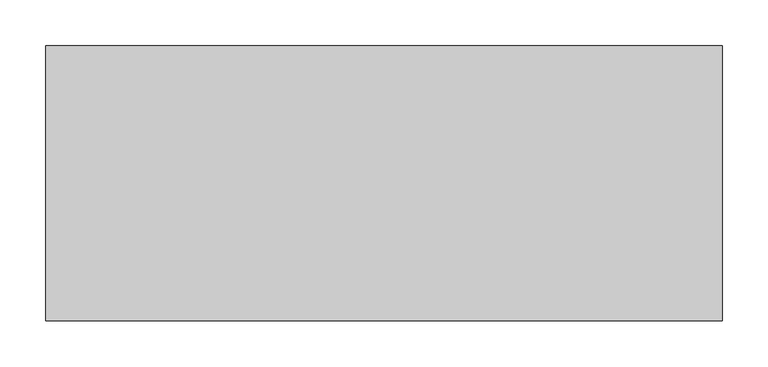
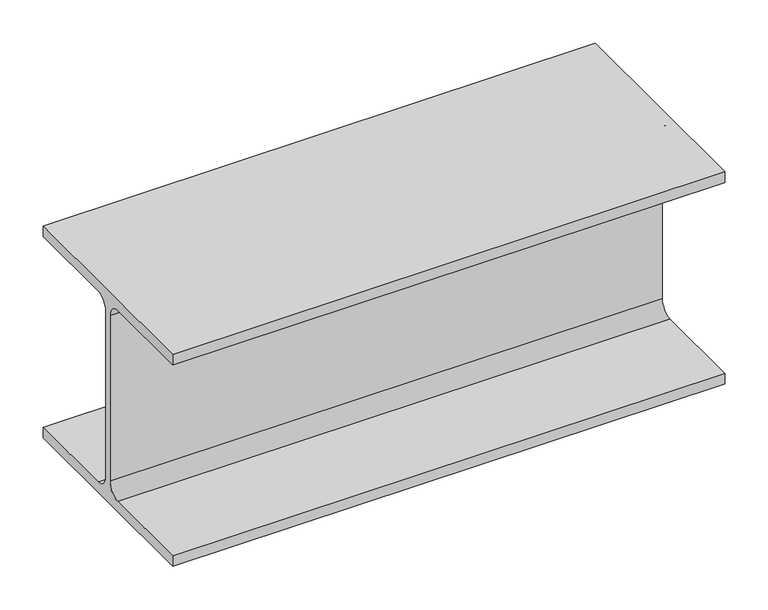
"""IFC4 building model written with IfcOpenShell, lengths in millimetres: beam geometry, 0912_Steel Framing_H-KSD3502 : H_SB_ASB_H-300x300x10x15."""

from ifc_helpers import new_model, si_unit, point, frame, frame_2d, origin, place, context, project, spatial, polyline, circle_curve, trimmed, segment, composite_curve, outline, extrude, source, transform, mapped, element, save


def beam_ee296e32(model_context):
    return source(origin(), model_context, "Body", "SweptSolid", [
        extrude(outline(composite_curve([segment(polyline([(150.0, -135.0), (150.0, -150.0), (-150.0, -150.0), (-150.0, -135.0), (-23.0, -135.0)]), True, "CONTINUOUS"), segment(trimmed(circle_curve(frame_2d((-23.0, -117.0)), 18.0), [point((-23.0, -135.0))], [point((-5.0, -117.0))], True, "CARTESIAN"), True, "CONTINUOUS"), segment(polyline([(-5.0, -117.0), (-5.0, 117.0)]), True, "CONTINUOUS"), segment(trimmed(circle_curve(frame_2d((-23.0, 117.0)), 18.0), [point((-5.0, 117.0))], [point((-23.0, 135.0))], True, "CARTESIAN"), True, "CONTINUOUS"), segment(polyline([(-23.0, 135.0), (-150.0, 135.0), (-150.0, 150.0), (150.0, 150.0), (150.0, 135.0), (23.0, 135.0)]), True, "CONTINUOUS"), segment(trimmed(circle_curve(frame_2d((23.0, 117.0)), 18.0), [point((23.0, 135.0))], [point((5.0, 117.0))], True, "CARTESIAN"), True, "CONTINUOUS"), segment(polyline([(5.0, 117.0), (5.0, -117.0)]), True, "CONTINUOUS"), segment(trimmed(circle_curve(frame_2d((23.0, -117.0)), 18.0), [point((5.0, -117.0))], [point((23.0, -135.0))], True, "CARTESIAN"), True, "CONTINUOUS"), segment(polyline([(23.0, -135.0), (150.0, -135.0)]), True, "CONTINUOUS")], self_intersect=False)), frame((-502.5, 0.0, 0.0), z_axis=(1.0, 0.0, 0.0), x_axis=(0.0, 1.0, 0.0)), (0.0, 0.0, 1.0), 738.1129602),
    ])


if __name__ == "__main__":
    model = new_model("IFC4")
    model_context = context("Model", 3, world=origin())
    ifc_project = project(units=[si_unit("LENGTHUNIT", "METRE", prefix="MILLI")], contexts=[model_context])
    site = spatial("IfcSite", under=ifc_project)
    building = spatial("IfcBuilding", under=site)
    placement = place(None, origin())
    beam_shape = beam_ee296e32(model_context)
    element("IfcBeam", 1, ObjectType="0912_Steel Framing_H-KSD3502 : H_SB_ASB_H-300x300x10x15", at=placement, inside=building, context=model_context, shape_type="MappedRepresentation", body=[
        mapped(beam_shape, transform((0.0, 0.0, 0.0), x_axis=(1.0, 0.0, 0.0), y_axis=(0.0, 1.0, 0.0), z_axis=(0.0, 0.0, 1.0))),
    ])
    save(model, "model.ifc")

# Revit data of these elements
# Type "0912_Steel Framing_H-KSD3502 : H_SB_ASB_H-300x300x10x15"
#   H_WM Code_1 = "S01AA001-00001 | Main Steel Structure Fabrication Work | Shelter/Building | Heavy Steel - Standard (Weight≥90KG/M) | Material: (   )"
#   H_WM Code_2 = "S03AA027-00001 | Main Steel Structure Erection Work | Shelter/Building | Heavy Steel (Weight≥90KG/M) | Material: (   )"
#   H_WM Code_3 = "S01AA010-00001 | Main Steel Structure Fabrication Work | Shelter/Building | Steel Painting/Coating | for Non-Fireproofed Steel Surface, Surface Preparation, Primer, Second & Final Coat | Material: (   )"
#   H_Q'ty Cal Type Tag = "SB-Q2"
#   Width = 30.0 cm
#   Web Thickness = 1.0 cm
#   Web Fillet = 1.8 cm
#   Warping Constant = 1370000.0 cm⁶
#   W = 0
#   Torsional Moment of Inertia = 77.00 cm⁴
#   Section Area = 119.8 cm²
#   Plastic Modulus weak axis = 684.0 cm³
#   Plastic Modulus strong axis = 1500.0 cm³
#   Perimeter = 1.75 m²/m
#   Nominal Weight = 94.00 kgf/m
#   Moment of Inertia weak axis = 6750.00 cm⁴
#   Moment of Inertia strong axis = 20400.00 cm⁴
#   Height = 30.0 cm
#   Flange Thickness = 1.5 cm
#   Elastic Modulus weak axis = 450.0 cm³
#   Elastic Modulus strong axis = 1360.0 cm³
#   Centroid Vertical = 15.0 cm
#   Centroid Horizontal = 15.0 cm
#   Ix = 204000000
#   Length [instance default] = 1.5240 m
#   Zx = 1500000
#   b = 0.3000 m
#   h = 0.3000 m
#   r = 0.0180 m
#   s = 0.0100 m
#   t = 0.0150 m
#   A = 0.01198 m²
#   Structural Material [instance default] = Steel, 45-345
#   Assembly Code = ""
# Element 1 (IfcBeam, "0912_Steel Framing_H-KSD3502 : H_SB_ASB_H-300x300x10x15")
#   Structural Material = none
# Materials
#   "Steel, 45-345": class "Metal", colour RGB 189 187 185, transparency 0, Description = "Steel 345 MPa", Cost = 0
